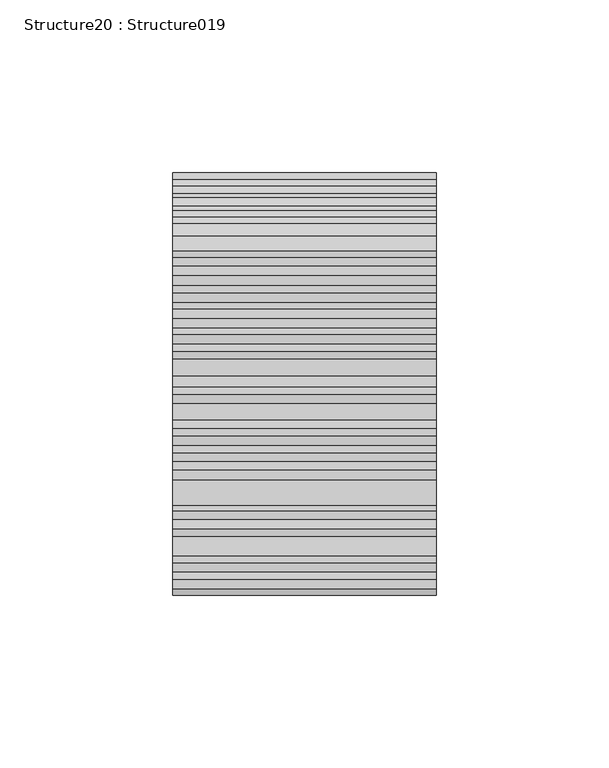
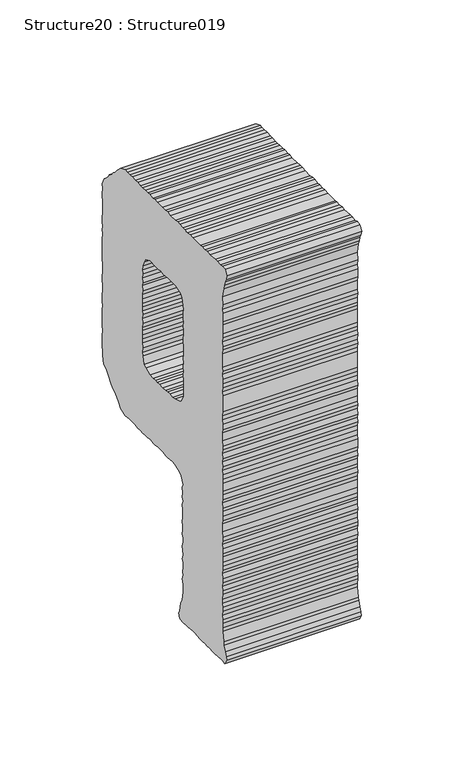
"""IFC4 building model written with IfcOpenShell, lengths in millimetres: proxy geometry, Structure20 : Structure019."""

import ifcopenshell
import ifcopenshell.guid

model = None  # the IFC model being written
_history = None  # IfcOwnerHistory: only IFC2X3 demands one
_inside = {}  # id of a spatial element -> (the spatial element, [elements in it])
_under = {}  # id of a project, library or spatial element -> (it, [spatial elements below it])
_declared = {}  # id of a project -> (the project, [libraries it declares])
_typed = {}  # id of a type object -> (the type object, [elements of that type])
_made_of = {}  # id of a material, layer set ... -> (it, [elements and type objects made of it])


def new_model(schema):
    """Start an empty IFC model of exactly this schema.

    Asked for "IFC4X3", IfcOpenShell would pick the latest addendum, in which some entities
    have other attributes; the version numbers below select the first issue.
    IFC2X3 requires an IfcOwnerHistory on every rooted entity: one is made here for all.
    """
    global model, _history
    if schema == "IFC4X3":
        model = ifcopenshell.file(schema_version=(4, 3, 0, 0))
    else:
        model = ifcopenshell.file(schema=schema)
    _inside.clear()
    _under.clear()
    _declared.clear()
    _typed.clear()
    _made_of.clear()
    _history = None
    if model.schema == "IFC2X3":
        org = make("IfcOrganization", Name="unknown")
        user = make(
            "IfcPersonAndOrganization",
            ThePerson=make("IfcPerson", FamilyName="unknown"),
            TheOrganization=org,
        )
        app = make(
            "IfcApplication",
            ApplicationDeveloper=org,
            Version="unknown",
            ApplicationFullName="unknown",
            ApplicationIdentifier="unknown",
        )
        _history = make(
            "IfcOwnerHistory",
            OwningUser=user,
            OwningApplication=app,
            ChangeAction="ADDED",
            CreationDate=0,
        )
    return model


def make(cls, **values):
    """One entity of the class cls with the attributes given. An attribute that is None is left unset."""
    return model.create_entity(
        cls, **{name: value for name, value in values.items() if value is not None}
    )


def rooted(cls, **values):
    """An entity with a GlobalId (a new one), such as an element, a storey or a relation."""
    return make(cls, GlobalId=ifcopenshell.guid.new(), OwnerHistory=_history, **values)


def si_unit(unit_type, name, prefix=None):
    """IfcSIUnit, for example si_unit("LENGTHUNIT", "METRE", prefix="MILLI")."""
    return make("IfcSIUnit", UnitType=unit_type, Prefix=prefix, Name=name)


def assignment(units):
    """IfcUnitAssignment: the units of a project."""
    return None if units is None else make("IfcUnitAssignment", Units=units)


def point(xyz):
    """IfcCartesianPoint."""
    return None if xyz is None else make("IfcCartesianPoint", Coordinates=xyz)


def direction(xyz):
    """IfcDirection."""
    return None if xyz is None else make("IfcDirection", DirectionRatios=xyz)


def frame(location, z_axis=None, x_axis=None):
    """IfcAxis2Placement3D, a coordinate frame: its origin and axes. An axis left out is left unset."""
    return make(
        "IfcAxis2Placement3D",
        Location=point(location),
        Axis=direction(z_axis),
        RefDirection=direction(x_axis),
    )


def origin():
    """The frame at (0, 0, 0) with its axes left unset."""
    return frame((0.0, 0.0, 0.0))


def place(relative_to, where):
    """IfcLocalPlacement: puts the frame where relative to a parent placement (None: the world)."""
    return make(
        "IfcLocalPlacement", PlacementRelTo=relative_to, RelativePlacement=where
    )


def context(
    kind, dimensions, precision=None, world=None, true_north=None, identifier=None
):
    """IfcGeometricRepresentationContext, for example the 3D "Model" context."""
    return make(
        "IfcGeometricRepresentationContext",
        ContextIdentifier=identifier,
        ContextType=kind,
        CoordinateSpaceDimension=dimensions,
        Precision=precision,
        WorldCoordinateSystem=world,
        TrueNorth=true_north,
    )


def project(units=None, contexts=None):
    """IfcProject with its units and contexts."""
    return rooted(
        "IfcProject",
        Name="project",
        RepresentationContexts=contexts,
        UnitsInContext=assignment(units),
    )


def spatial(cls, under=None, at=None, **own):
    """A site, building, storey or space (cls), placed at a placement, below another one or the project."""
    s = rooted(cls, ObjectPlacement=at, **own)
    if under is not None:
        _under.setdefault(under.id(), (under, []))[1].append(s)
    return s


def polyline(points):
    """IfcPolyline through the points."""
    return make("IfcPolyline", Points=[point(p) for p in points])


def outline(outer, holes=None, kind="AREA"):
    """IfcArbitraryClosedProfileDef: a profile drawn as a closed curve; with holes, ...WithVoids."""
    if holes is None:
        return make("IfcArbitraryClosedProfileDef", ProfileType=kind, OuterCurve=outer)
    return make(
        "IfcArbitraryProfileDefWithVoids",
        ProfileType=kind,
        OuterCurve=outer,
        InnerCurves=holes,
    )


def extrude(swept, where, along, depth):
    """IfcExtrudedAreaSolid: the profile swept, set in the frame where, extruded along a direction by depth."""
    return make(
        "IfcExtrudedAreaSolid",
        SweptArea=swept,
        Position=where,
        ExtrudedDirection=direction(along),
        Depth=depth,
    )


def shape(context_of_items, identifier, shape_type, items):
    """IfcShapeRepresentation: the items that make up one representation, for example the "Body"."""
    return make(
        "IfcShapeRepresentation",
        ContextOfItems=context_of_items,
        RepresentationIdentifier=identifier,
        RepresentationType=shape_type,
        Items=items,
    )


def source(mapping_origin, context_of_items, identifier, shape_type, items):
    """IfcRepresentationMap: a shape defined once, which mapped items show again and again."""
    return make(
        "IfcRepresentationMap",
        MappingOrigin=mapping_origin,
        MappedRepresentation=shape(context_of_items, identifier, shape_type, items),
    )


def transform(
    local_origin,
    x_axis=None,
    y_axis=None,
    z_axis=None,
    scale=None,
    scale2=None,
    scale3=None,
    uniform=True,
):
    """IfcCartesianTransformationOperator3D, or its non-uniform kind. x_axis, y_axis, z_axis: its Axis1, 2, 3."""
    if uniform:
        return make(
            "IfcCartesianTransformationOperator3D",
            Axis1=direction(x_axis),
            Axis2=direction(y_axis),
            LocalOrigin=point(local_origin),
            Scale=scale,
            Axis3=direction(z_axis),
        )
    return make(
        "IfcCartesianTransformationOperator3DnonUniform",
        Axis1=direction(x_axis),
        Axis2=direction(y_axis),
        LocalOrigin=point(local_origin),
        Scale=scale,
        Axis3=direction(z_axis),
        Scale2=scale2,
        Scale3=scale3,
    )


def mapped(mapping_source, mapping_target):
    """IfcMappedItem: shows the shape of a source again, moved by a transform."""
    return make(
        "IfcMappedItem", MappingSource=mapping_source, MappingTarget=mapping_target
    )


def made_of(thing, what):
    """Note that an element or type object is made of a material, layer set ...; save() writes the relation."""
    if what is not None:
        _made_of.setdefault(what.id(), (what, []))[1].append(thing)
    return thing


def element(
    cls,
    number,
    at=None,
    inside=None,
    cuts=None,
    type_object=None,
    material=None,
    context=None,
    identifier="Body",
    shape_type=None,
    held_by="IfcProductDefinitionShape",
    body=None,
    shapes=None,
    **own,
):
    """One element of the class cls, such as IfcWall. Its Tag is "e" and its number.

    at: its placement. inside: the storey or other place that contains it. cuts: it is an
    opening in that element (IfcRelVoidsElement). A single representation is given by context,
    identifier, shape_type and body (its items); several are given by shapes. held_by: the class
    of the entity that holds the representations. save() writes the other relations.
    """
    e = rooted(cls, Tag="e%d" % number, ObjectPlacement=at, **own)
    if body is not None:
        shapes = [shape(context, identifier, shape_type, body)]
    if shapes is not None:
        e.Representation = make(held_by, Representations=shapes)
    if inside is not None:
        _inside.setdefault(inside.id(), (inside, []))[1].append(e)
    if cuts is not None:
        rooted(
            "IfcRelVoidsElement", RelatingBuildingElement=cuts, RelatedOpeningElement=e
        )
    if type_object is not None:
        _typed.setdefault(type_object.id(), (type_object, []))[1].append(e)
    return made_of(e, material)


def aggregate(whole, parts):
    """IfcRelAggregates: a whole, such as a stair, and the parts it consists of."""
    return rooted("IfcRelAggregates", RelatingObject=whole, RelatedObjects=parts)


def save(model, path):
    """Write the relations noted so far, then the file.

    IfcRelAggregates (storeys below a building ...), IfcRelContainedInSpatialStructure (elements
    in a storey), IfcRelDefinesByType, IfcRelAssociatesMaterial and IfcRelDeclares: one each for
    every whole, place, type object, material and project.
    """
    for whole, parts in _under.values():
        aggregate(whole, parts)
    for where, things in _inside.values():
        rooted(
            "IfcRelContainedInSpatialStructure",
            RelatedElements=things,
            RelatingStructure=where,
        )
    for kind, things in _typed.values():
        rooted("IfcRelDefinesByType", RelatedObjects=things, RelatingType=kind)
    for what, things in _made_of.values():
        rooted("IfcRelAssociatesMaterial", RelatedObjects=things, RelatingMaterial=what)
    for by, libraries in _declared.values():
        rooted("IfcRelDeclares", RelatingContext=by, RelatedDefinitions=libraries)
    model.write(path)


def structure20_structure019_c485a753(model_context):
    return source(origin(), model_context, "Body", "SweptSolid", [
        extrude(outline(polyline([(4.6417015, 0.0), (7.4229948, 0.6116643), (9.5917767, 0.3032906), (12.6899155, 0.0), (17.6357547, 0.0), (19.8003007, 0.6116643), (21.9648467, 0.0), (24.7546118, 0.6116643), (26.6073954, 0.3032906), (29.3878415, 0.3032906), (32.1776066, 0.0), (34.0303902, 0.0), (36.8201553, 0.3032906), (38.9762294, 0.3032906), (41.7659946, 0.6116643), (44.5506766, 0.3032906), (47.0235962, 0.3032906), (48.8763798, 0.6116643), (53.2105548, -1.2495911), (56.9195107, -4.6518676), (58.7765301, -6.8164136), (60.6335496, -8.3565876), (61.8746689, -9.9103165), (64.3467414, -11.7571698), (65.5836248, -13.6285913), (67.7481708, -15.7787352), (69.6060374, -17.3324641), (71.4622097, -21.3591126), (70.8412265, -24.1353229), (71.4622097, -26.9115331), (71.4622097, -28.7821075), (70.8412265, -31.5574705), (70.8412265, -38.6780219), (71.4622097, -41.1509415), (71.4622097, -44.2439973), (70.8412265, -46.4220981), (71.153836, -48.5730892), (70.8412265, -51.046856), (71.153836, -54.1526194), (71.4622097, -56.3180126), (71.4622097, -58.7773773), (71.153836, -61.2587687), (71.4622097, -64.3518244), (71.153836, -66.8255913), (70.8412265, -68.9994562), (70.8412265, -73.9546145), (71.4622097, -76.4122849), (71.4622097, -79.20205), (70.8412265, -81.6851358), (70.8412265, -83.5319891), (71.4622097, -89.1072834), (71.153836, -91.8885767), (70.8412265, -93.7455962), (71.4622097, -96.8386519), (71.153836, -98.9947261), (71.4622097, -101.4761175), (71.4622097, -103.9490371), (71.153836, -106.1144303), (70.8412265, -108.8991123), (71.153836, -111.6897246), (71.4622097, -114.1617971), (71.4622097, -118.4917362), (70.8412265, -120.9739748), (70.8412265, -123.4418113), (69.9177998, -128.3876506), (67.4406443, -129.6330058), (66.2037609, -131.4807063), (62.494805, -135.8097982), (60.9410761, -137.3635271), (58.4732396, -138.6004105), (55.3751008, -142.3051305), (53.2105548, -144.7865219), (48.8763798, -146.3309318), (47.0235962, -146.0234054), (44.2431501, -145.7057127), (38.9762294, -145.7057127), (36.5075457, -146.3309318), (34.0303902, -146.0234054), (31.5532346, -146.3309318), (29.7004511, -146.0234054), (26.6073954, -146.0234054), (24.4428494, -145.7057127), (21.6573202, -146.3309318), (19.8003007, -146.0234054), (16.7114809, -145.7057127), (12.0646963, -145.7057127), (9.2791671, -146.3309318), (7.118857, -146.0234054), (4.9543111, -146.0234054), (2.4771555, -145.7057127), (-0.6167473, -146.3309318), (-4.6425487, -147.5627322), (-5.874349, -149.1164611), (-7.7313685, -153.1431096), (-7.1103852, -155.3076555), (-7.4229948, -158.3913923), (-7.1103852, -160.8736309), (-7.7313685, -163.0381768), (-7.1103852, -165.20357), (-7.4229948, -168.2966257), (-7.4229948, -172.9434103), (-7.1103852, -175.4163299), (-7.4229948, -177.8892496), (-7.4229948, -180.3570861), (-7.1103852, -183.1468512), (-7.7313685, -185.0038707), (-7.7313685, -187.7843168), (-7.1103852, -190.2530006), (-7.4229948, -193.0520847), (-7.7313685, -195.2073116), (-7.1103852, -197.9970768), (-7.7313685, -199.8540962), (-7.7313685, -202.3270159), (-7.4229948, -205.4065167), (-7.7313685, -207.277091), (-7.1103852, -209.7500107), (-7.7313685, -212.8430664), (-7.7313685, -217.4813792), (-7.1103852, -222.4356902), (-5.5668225, -225.5151911), (-4.6425487, -230.4703493), (-3.4014294, -232.3316047), (-4.6425487, -234.7994412), (-7.1103852, -235.4246604), (-12.37307, -235.4246604), (-15.1543633, -235.1171339), (-17.3189093, -234.7994412), (-19.1759287, -234.7994412), (-24.7419041, -235.4246604), (-26.9115331, -235.4246604), (-29.3844528, -235.1171339), (-31.5532346, -235.4246604), (-34.0261543, -235.1171339), (-36.8074476, -235.4246604), (-39.2846031, -235.4246604), (-41.1416226, -235.1171339), (-46.3992243, -235.1171339), (-48.5646174, -235.4246604), (-50.4165538, -232.3316047), (-49.8057367, -230.4703493), (-48.8721439, -228.0016656), (-47.6403436, -224.9035268), (-47.327734, -223.0473545), (-46.3992243, -217.4813792), (-46.3992243, -215.315986), (-46.7075979, -212.5397758), (-46.7075979, -210.3616749), (-46.0916978, -207.8929912), (-46.7075979, -205.1125451), (-46.7075979, -202.9386801), (-46.0916978, -200.782606), (-46.0916978, -198.3012145), (-46.3992243, -195.2073116), (-46.3992243, -193.0520847), (-46.0916978, -190.569846), (-46.3992243, -188.4053001), (-46.7075979, -185.9230614), (-46.0916978, -182.8300057), (-46.7075979, -180.6739316), (-46.7075979, -178.5000666), (-46.3992243, -176.027147), (-46.3992243, -172.9434103), (-46.7075979, -170.7695453), (-46.3992243, -167.9933351), (-46.0916978, -165.5204155), (-46.3992243, -163.663396), (-46.3992243, -161.1904764), (-46.0916978, -158.0838658), (-46.0916978, -153.4464002), (-46.3992243, -151.281007), (-46.7075979, -148.496325), (-46.3992243, -145.7057127), (-46.3992243, -143.8580122), (-46.0916978, -140.7649565), (-46.7075979, -138.6004105), (-46.3992243, -135.8097982), (-46.7075979, -133.6588072), (-46.7075979, -128.7044961), (-46.3992243, -126.5255481), (-46.3992243, -123.7493378), (-46.0916978, -121.2772654), (-46.7075979, -118.7950268), (-46.0916978, -116.326343), (-46.7075979, -114.1617971), (-46.0916978, -111.0645055), (-46.7075979, -108.5958217), (-46.3992243, -106.7345663), (-46.0916978, -103.6415106), (-46.0916978, -98.9947261), (-46.7075979, -96.8386519), (-46.3992243, -93.7455962), (-46.0916978, -91.2625104), (-46.0916978, -88.7904379), (-46.3992243, -86.3217542), (-46.3992243, -76.7299775), (-46.0916978, -74.5561126), (-46.7075979, -71.7756664), (-46.3992243, -69.6102733), (-46.7075979, -66.5172176), (-46.0916978, -64.049381), (-46.3992243, -61.8848351), (-46.0916978, -59.715206), (-46.0916978, -51.6669921), (-46.3992243, -49.1983083), (-46.3992243, -47.3362058), (-46.0916978, -44.5515237), (-46.7075979, -41.7710776), (-46.3992243, -39.6056845), (-46.3992243, -34.3472356), (-46.7075979, -32.1835368), (-46.7075979, -27.2292258), (-46.0916978, -25.0638326), (-46.7075979, -21.9843318), (-46.0916978, -17.6408378), (-47.327734, -12.0748625), (-48.2520078, -9.6019428), (-48.8721439, -7.1332591), (-49.8057367, -5.2720037), (-50.7291634, -2.4864745), (-48.8721439, 0.3032906), (-46.0916978, 0.6116643), (-43.9263046, 0.0), (-41.4491491, 0.6116643), (-39.2846031, 0.6116643), (-33.7186278, 0.0), (-31.5532346, 0.6116643), (-28.7634695, 0.0), (-26.295633, 0.3032906), (-24.7419041, 0.0), (-17.3189093, 0.0), (-14.5384631, 0.3032906), (-12.0655435, 0.0), (-9.588388, 0.3032906), (-7.4229948, 0.0), (-4.6425487, 0.6116643), (-2.4729196, 0.6116643), (0.0, 0.0), (4.6417015, 0.0)]), holes=[polyline([(-4.9458393, -105.1943923), (0.0, -106.7345663), (2.1687819, -107.04294), (4.9543111, -106.7345663), (7.4229948, -107.04294), (9.2791671, -107.04294), (12.0646963, -107.3453834), (14.8544614, -107.04294), (17.3231452, -107.3453834), (19.1801646, -107.04294), (21.6573202, -107.3453834), (24.4428494, -107.04294), (28.1518053, -105.1943923), (30.3214343, -104.2658826), (31.244861, -99.9367907), (31.864997, -98.0755353), (31.244861, -94.9824796), (31.864997, -92.5087128), (31.864997, -90.040029), (31.5532346, -87.5544017), (31.864997, -85.085718), (31.5532346, -82.9076171), (31.244861, -80.4389334), (31.864997, -77.9668609), (31.244861, -75.1770958), (31.864997, -73.3285481), (31.5532346, -70.8471567), (31.5532346, -68.6817636), (31.864997, -66.2130798), (31.864997, -63.4233147), (31.244861, -60.9512423), (31.864997, -58.1741848), (31.244861, -56.3180126), (31.5532346, -53.5282474), (31.244861, -50.7384823), (31.5532346, -48.5730892), (31.244861, -46.1060998), (29.7004511, -42.7038233), (28.7770244, -40.8425679), (24.7546118, -39.2896862), (19.8003007, -39.2896862), (16.7114809, -39.6056845), (14.5418519, -38.9855484), (11.7571698, -39.6056845), (9.9001504, -39.2896862), (7.4229948, -38.9855484), (-0.3083737, -38.9855484), (-4.9458393, -40.5392773), (-6.4944851, -42.3954496), (-7.4229948, -46.1060998), (-7.7313685, -48.5730892), (-7.4229948, -51.046856), (-7.4229948, -53.8459401), (-8.038895, -56.3180126), (-7.4229948, -58.1741848), (-7.7313685, -61.2587687), (-8.038895, -63.4233147), (-7.4229948, -65.9064005), (-7.4229948, -68.0709465), (-7.7313685, -70.529464), (-7.7313685, -75.4837751), (-7.4229948, -78.2837064), (-7.7313685, -80.1322541), (-7.4229948, -82.9076171), (-7.7313685, -85.7117843), (-7.4229948, -87.8627754), (-8.038895, -90.6381384), (-7.7313685, -92.5087128), (-8.038895, -94.9824796), (-7.7313685, -98.0755353), (-7.7313685, -100.5476078), (-6.1869586, -103.9490371), (-4.9458393, -105.1943923)])]), frame((-35624.0862846, 274894.4692333, 4217.9376236), z_axis=(1.0, 0.0, 1.354250045437766e-12), x_axis=(0.0, 1.0, 0.0)), (0.0, 0.0, 1.0), 76.2),
    ])


if __name__ == "__main__":
    model = new_model("IFC4")
    model_context = context("Model", 3, world=origin())
    ifc_project = project(units=[si_unit("LENGTHUNIT", "METRE", prefix="MILLI")], contexts=[model_context])
    site = spatial("IfcSite", under=ifc_project)
    building = spatial("IfcBuilding", under=site)
    placement = place(None, origin())
    structure20_structure019_shape = structure20_structure019_c485a753(model_context)
    element("IfcBuildingElementProxy", 1, Name="Structure20 : Structure019", ObjectType="Structure20 : Structure019", at=placement, inside=building, context=model_context, shape_type="MappedRepresentation", body=[
        mapped(structure20_structure019_shape, transform((0.0, 0.0, 0.0), x_axis=(1.0, 0.0, 0.0), y_axis=(0.0, 1.0, 0.0), z_axis=(0.0, 0.0, 1.0))),
    ])
    save(model, "model.ifc")

# Revit data of these elements
# Type "Structure20 : Structure019"
#   NameOverride = "Structure019"
# Element 1 (IfcBuildingElementProxy, "Structure20 : Structure019")
#   Materials on its faces: "BRUSHED ALUMINUM LETTERING"
# Materials
#   "BRUSHED ALUMINUM LETTERING": class "Unassigned", colour RGB 169 181 186, transparency 0, Cost = 0
